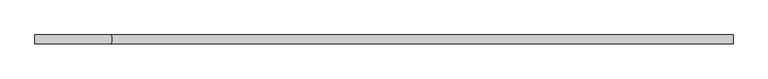
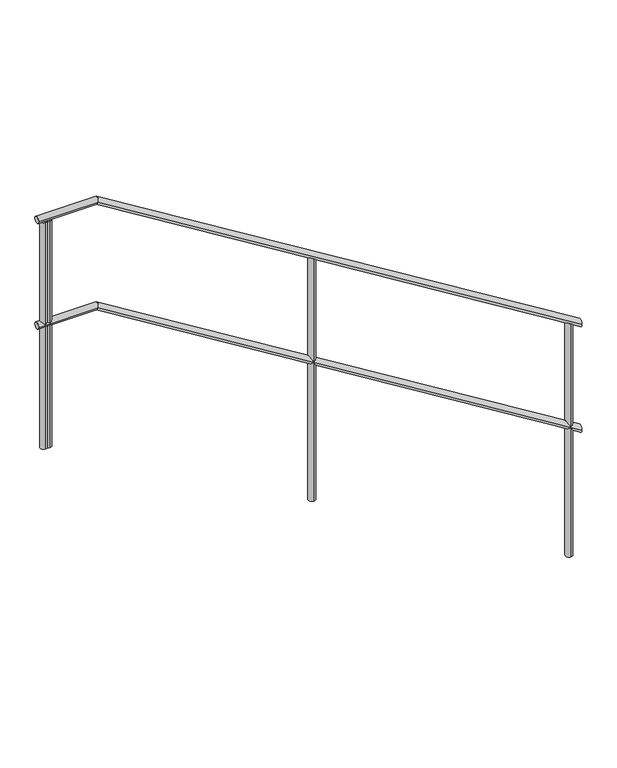
"""IFC4 building model written with IfcOpenShell, lengths in millimetres: railing geometry."""

from ifc_helpers import new_model, si_unit, point, frame, frame_2d, origin, place, context, project, spatial, circle_curve, ellipse_curve, trimmed, segment, composite_curve, outline, extrude, source, transform, mapped, element, save
from ifc_brep_helpers import plane_surface, cylinder_surface, advanced_brep


def railing_ad897b6d(model_context):
    return source(origin(), model_context, "Body", "SolidModel", [
        advanced_brep(
        [(6405.7243044, 65167.0208589, -450.9609787), (6405.7243044, 65137.0208589, -450.9609787), (4241.4675189, 65167.0208589, 885.0), (4241.4675189, 65137.0208589, 885.0), (3975.7243044, 65167.0208589, 885.0), (3975.7243044, 65137.0208589, 885.0)],
        [
            (0, 1, ellipse_curve(frame((6405.7243044, 65152.0208589, -450.9609787), z_axis=(1.0, 0.0, 0.0), x_axis=(0.0, 0.0, -1.0)), 17.6276454, 15.0)),
            (1, 0, ellipse_curve(frame((6405.7243044, 65152.0208589, -450.9609787), z_axis=(1.0, 0.0, 0.0), x_axis=(0.0, 0.0, -1.0)), 17.6276454, 15.0)),
            (0, 2),
            (2, 3, ellipse_curve(frame((4241.4675189, 65152.0208589, 885.0), z_axis=(0.9620125025549408, 0.0, -0.2730053935877092), x_axis=(-0.2730053935877087, 0.0, -0.962012502554941)), 15.5923129, 15.0)),
            (3, 1),
            (3, 2, ellipse_curve(frame((4241.4675189, 65152.0208589, 885.0), z_axis=(0.9620125025549408, 0.0, -0.2730053935877092), x_axis=(-0.2730053935877087, 0.0, -0.962012502554941)), 15.5923129, 15.0)),
            (4, 5, circle_curve(frame((3975.7243044, 65152.0208589, 885.0), z_axis=(-1.0, 0.0, 0.0), x_axis=(0.0, -1.0, 0.0)), 15.0)),
            (5, 4, circle_curve(frame((3975.7243044, 65152.0208589, 885.0), z_axis=(-1.0, 0.0, 0.0), x_axis=(0.0, -1.0, 0.0)), 15.0)),
            (2, 4),
            (5, 3),
        ],
        [
            plane_surface(frame((6405.7243044, 65152.0208589, -433.3333333), z_axis=(1.0, 0.0, 0.0), x_axis=(0.0, -1.0, 0.0))),
            cylinder_surface(frame((6397.8452664, 65152.0208589, -446.097375), z_axis=(0.8509361101440399, 0.0, -0.5252692037926174), x_axis=(0.0, -1.0, 0.0)), 15.0),
            plane_surface(frame((3975.7243044, 65152.0208589, 900.0), z_axis=(-1.0, 0.0, 0.0), x_axis=(0.0, -1.0, 0.0))),
            cylinder_surface(frame((4245.7243044, 65152.0208589, 885.0), z_axis=(1.0, 0.0, 0.0), x_axis=(0.0, -1.0, 0.0)), 15.0),
        ],
        [
            (0, [[1, 2]]),
            (1, [[-1, 3, 4, 5]]),
            (1, [[-2, -5, 6, -3]]),
            (2, [[7, 8]]),
            (3, [[-4, 9, -8, 10]]),
            (3, [[-6, -10, -7, -9]]),
        ],
    ),
        advanced_brep(
        [(6405.7243044, 65167.0208589, 49.0390213), (6405.7243044, 65137.0208589, 49.0390213), (4241.4675189, 65167.0208589, 1385.0), (4241.4675189, 65137.0208589, 1385.0), (3975.7243044, 65167.0208589, 1385.0), (3975.7243044, 65137.0208589, 1385.0)],
        [
            (0, 1, ellipse_curve(frame((6405.7243044, 65152.0208589, 49.0390213), z_axis=(1.0, 0.0, 0.0), x_axis=(0.0, 0.0, -1.0)), 17.6276454, 15.0)),
            (1, 0, ellipse_curve(frame((6405.7243044, 65152.0208589, 49.0390213), z_axis=(1.0, 0.0, 0.0), x_axis=(0.0, 0.0, -1.0)), 17.6276454, 15.0)),
            (0, 2),
            (2, 3, ellipse_curve(frame((4241.4675189, 65152.0208589, 1385.0), z_axis=(0.9620125025549408, 0.0, -0.2730053935877092), x_axis=(-0.2730053935877087, 0.0, -0.962012502554941)), 15.5923129, 15.0)),
            (3, 1),
            (3, 2, ellipse_curve(frame((4241.4675189, 65152.0208589, 1385.0), z_axis=(0.9620125025549408, 0.0, -0.2730053935877092), x_axis=(-0.2730053935877087, 0.0, -0.962012502554941)), 15.5923129, 15.0)),
            (4, 5, circle_curve(frame((3975.7243044, 65152.0208589, 1385.0), z_axis=(-1.0, 0.0, 0.0), x_axis=(0.0, -1.0, 0.0)), 15.0)),
            (5, 4, circle_curve(frame((3975.7243044, 65152.0208589, 1385.0), z_axis=(-1.0, 0.0, 0.0), x_axis=(0.0, -1.0, 0.0)), 15.0)),
            (2, 4),
            (5, 3),
        ],
        [
            plane_surface(frame((6405.7243044, 65152.0208589, 66.6666667), z_axis=(1.0, 0.0, 0.0), x_axis=(0.0, -1.0, 0.0))),
            cylinder_surface(frame((6397.8452664, 65152.0208589, 53.902625), z_axis=(0.8509361101440399, 0.0, -0.5252692037926174), x_axis=(0.0, -1.0, 0.0)), 15.0),
            plane_surface(frame((3975.7243044, 65152.0208589, 1400.0), z_axis=(-1.0, 0.0, 0.0), x_axis=(0.0, -1.0, 0.0))),
            cylinder_surface(frame((4245.7243044, 65152.0208589, 1385.0), z_axis=(1.0, 0.0, 0.0), x_axis=(0.0, -1.0, 0.0)), 15.0),
        ],
        [
            (0, [[1, 2]]),
            (1, [[-1, 3, 4, 5]]),
            (1, [[-2, -5, 6, -3]]),
            (2, [[7, 8]]),
            (3, [[-4, 9, -8, 10]]),
            (3, [[-6, -10, -7, -9]]),
        ],
    ),
        extrude(outline(composite_curve([segment(trimmed(circle_curve(frame_2d((4005.7243044, 65152.0208589)), 15.0), [point((4005.7243044, 65167.0208589))], [point((4005.7243044, 65137.0208589))], False, "CARTESIAN"), True, "CONTINUOUS"), segment(trimmed(circle_curve(frame_2d((4005.7243044, 65152.0208589)), 15.0), [point((4005.7243044, 65137.0208589))], [point((4005.7243044, 65167.0208589))], False, "CARTESIAN"), True, "CONTINUOUS")], self_intersect=False)), frame((0.0, 0.0, 300.0), z_axis=(0.0, 0.0, 1.0), x_axis=(1.0, 0.0, 0.0)), (0.0, 0.0, 1.0), 1070.0),
        advanced_brep(
        [(5205.7243044, 65137.0208589, 777.4074074), (5205.7243044, 65167.0208589, 777.4074074), (5205.7243044, 65167.0208589, -366.6666667), (5205.7243044, 65137.0208589, -366.6666667)],
        [
            (0, 1, ellipse_curve(frame((5205.7243044, 65152.0208589, 777.4074074), z_axis=(-0.5252692037926167, 0.0, -0.8509361101440406), x_axis=(-0.8509361101440406, 0.0, 0.5252692037926162)), 17.6276454, 15.0)),
            (1, 2),
            (2, 3, circle_curve(frame((5205.7243044, 65152.0208589, -366.6666667), z_axis=(0.0, 0.0, 1.0), x_axis=(0.0, 1.0, 0.0)), 15.0)),
            (3, 0),
            (3, 2, circle_curve(frame((5205.7243044, 65152.0208589, -366.6666667), z_axis=(0.0, 0.0, 1.0), x_axis=(0.0, 1.0, 0.0)), 15.0)),
            (1, 0, ellipse_curve(frame((5205.7243044, 65152.0208589, 777.4074074), z_axis=(-0.5252692037926167, 0.0, -0.8509361101440406), x_axis=(-0.8509361101440406, 0.0, 0.5252692037926162)), 17.6276454, 15.0)),
        ],
        [
            cylinder_surface(frame((5205.7243044, 65152.0208589, -466.6666667), z_axis=(0.0, 0.0, 1.0), x_axis=(0.0, 1.0, 0.0)), 15.0),
            plane_surface(frame((5180.7243044, 65177.0208589, 792.8395062), z_axis=(0.5252692037926167, 0.0, 0.8509361101440406), x_axis=(0.0, -1.0, 0.0))),
            plane_surface(frame((5230.7243044, 65177.0208589, -366.6666667), z_axis=(0.0, 0.0, -1.0), x_axis=(0.0, -1.0, 0.0))),
        ],
        [
            (0, [[1, 2, 3, 4]]),
            (0, [[5, -2, 6, -4]]),
            (1, [[-6, -1]]),
            (2, [[-5, -3]]),
        ],
    ),
        extrude(outline(composite_curve([segment(trimmed(circle_curve(frame_2d((4025.7243044, 65152.0208589)), 15.0), [point((4025.7243044, 65167.0208589))], [point((4025.7243044, 65137.0208589))], False, "CARTESIAN"), True, "CONTINUOUS"), segment(trimmed(circle_curve(frame_2d((4025.7243044, 65152.0208589)), 15.0), [point((4025.7243044, 65137.0208589))], [point((4025.7243044, 65167.0208589))], False, "CARTESIAN"), True, "CONTINUOUS")], self_intersect=False)), frame((0.0, 0.0, 300.0), z_axis=(0.0, 0.0, 1.0), x_axis=(1.0, 0.0, 0.0)), (0.0, 0.0, 1.0), 1070.0),
        advanced_brep(
        [(6355.7243044, 65137.0208589, 67.5308642), (6355.7243044, 65167.0208589, 67.5308642), (6355.7243044, 65167.0208589, -1033.3333333), (6355.7243044, 65137.0208589, -1033.3333333)],
        [
            (0, 1, ellipse_curve(frame((6355.7243044, 65152.0208589, 67.5308642), z_axis=(-0.5252692037926167, 0.0, -0.8509361101440406), x_axis=(-0.8509361101440406, 0.0, 0.5252692037926162)), 17.6276454, 15.0)),
            (1, 2),
            (2, 3, circle_curve(frame((6355.7243044, 65152.0208589, -1033.3333333), z_axis=(0.0, 0.0, 1.0), x_axis=(0.0, 1.0, 0.0)), 15.0)),
            (3, 0),
            (3, 2, circle_curve(frame((6355.7243044, 65152.0208589, -1033.3333333), z_axis=(0.0, 0.0, 1.0), x_axis=(0.0, 1.0, 0.0)), 15.0)),
            (1, 0, ellipse_curve(frame((6355.7243044, 65152.0208589, 67.5308642), z_axis=(-0.5252692037926167, 0.0, -0.8509361101440406), x_axis=(-0.8509361101440406, 0.0, 0.5252692037926162)), 17.6276454, 15.0)),
        ],
        [
            cylinder_surface(frame((6355.7243044, 65152.0208589, -1133.3333333), z_axis=(0.0, 0.0, 1.0), x_axis=(0.0, 1.0, 0.0)), 15.0),
            plane_surface(frame((6330.7243044, 65177.0208589, 82.962963), z_axis=(0.5252692037926167, 0.0, 0.8509361101440406), x_axis=(0.0, -1.0, 0.0))),
            plane_surface(frame((6380.7243044, 65177.0208589, -1033.3333333), z_axis=(0.0, 0.0, -1.0), x_axis=(0.0, -1.0, 0.0))),
        ],
        [
            (0, [[1, 2, 3, 4]]),
            (0, [[5, -2, 6, -4]]),
            (1, [[-6, -1]]),
            (2, [[-5, -3]]),
        ],
    ),
    ])


if __name__ == "__main__":
    model = new_model("IFC4")
    model_context = context("Model", 3, world=origin())
    ifc_project = project(units=[si_unit("LENGTHUNIT", "METRE", prefix="MILLI")], contexts=[model_context])
    site = spatial("IfcSite", under=ifc_project)
    building = spatial("IfcBuilding", under=site)
    placement = place(None, origin())
    railing_shape = railing_ad897b6d(model_context)
    element("IfcRailing", 1, at=placement, inside=building, context=model_context, shape_type="MappedRepresentation", body=[
        mapped(railing_shape, transform((0.0, 0.0, 0.0), x_axis=(1.0, 0.0, 0.0), y_axis=(0.0, 1.0, 0.0), z_axis=(0.0, 0.0, 1.0))),
    ])
    save(model, "model.ifc")
